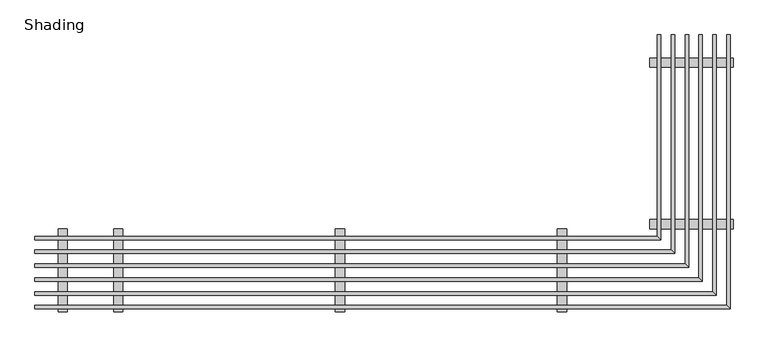
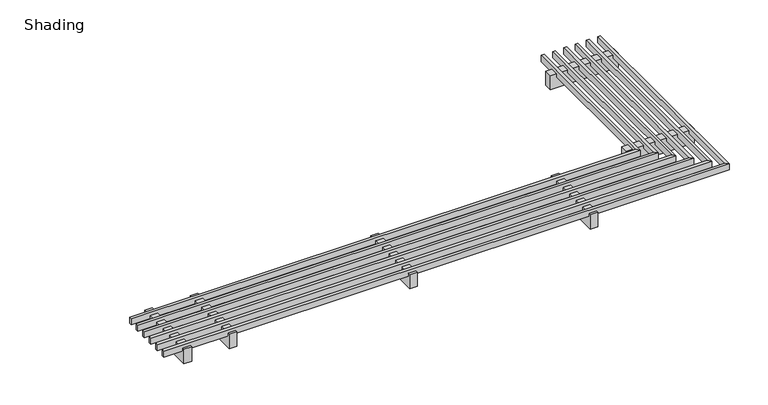
"""IFC4 building model written with IfcOpenShell, lengths in millimetres: railing geometry, Shading."""

from ifc_helpers import new_model, si_unit, frame, origin, place, context, project, spatial, polyline, outline, extrude, faceted_brep, source, transform, mapped, element, save


def shading_4c73cd6e(model_context):
    return source(origin(), model_context, "Body", "SolidModel", [
        faceted_brep([(-10644.3922358, -6454.4297826, 3702.05), (-10644.3922358, -6416.3297826, 3702.05), (-10644.3922358, -6416.3297826, 3613.15), (-10644.3922358, -6454.4297826, 3613.15), (-3005.3422358, -6454.4297826, 3613.15), (-3005.3422358, -6454.4297826, 3702.05), (-3043.4422358, -6416.3297826, 3613.15), (-3043.4422358, -6416.3297826, 3702.05), (-3005.3422358, -3438.1797826, 3702.05), (-3005.3422358, -3438.1797826, 3613.15), (-3043.4422358, -3438.1797826, 3613.15), (-3043.4422358, -3438.1797826, 3702.05)], [[[0, 1, 2, 3]], [[4, 5, 0, 3]], [[6, 4, 3, 2]], [[7, 6, 2, 1]], [[5, 7, 1, 0]], [[8, 9, 10, 11]], [[9, 8, 5, 4]], [[10, 9, 4, 6]], [[11, 10, 6, 7]], [[8, 11, 7, 5]]]),
        faceted_brep([(-10644.3922358, -6302.0297826, 3702.05), (-10644.3922358, -6263.9297826, 3702.05), (-10644.3922358, -6263.9297826, 3613.15), (-10644.3922358, -6302.0297826, 3613.15), (-3157.7422358, -6302.0297826, 3613.15), (-3157.7422358, -6302.0297826, 3702.05), (-3195.8422358, -6263.9297826, 3613.15), (-3195.8422358, -6263.9297826, 3702.05), (-3157.7422358, -3438.1797826, 3702.05), (-3157.7422358, -3438.1797826, 3613.15), (-3195.8422358, -3438.1797826, 3613.15), (-3195.8422358, -3438.1797826, 3702.05)], [[[0, 1, 2, 3]], [[4, 5, 0, 3]], [[6, 4, 3, 2]], [[7, 6, 2, 1]], [[5, 7, 1, 0]], [[8, 9, 10, 11]], [[9, 8, 5, 4]], [[10, 9, 4, 6]], [[11, 10, 6, 7]], [[8, 11, 7, 5]]]),
        faceted_brep([(-10644.3922358, -6149.6297826, 3702.05), (-10644.3922358, -6111.5297826, 3702.05), (-10644.3922358, -6111.5297826, 3613.15), (-10644.3922358, -6149.6297826, 3613.15), (-3310.1422358, -6149.6297826, 3613.15), (-3310.1422358, -6149.6297826, 3702.05), (-3348.2422358, -6111.5297826, 3613.15), (-3348.2422358, -6111.5297826, 3702.05), (-3310.1422358, -3438.1797826, 3702.05), (-3310.1422358, -3438.1797826, 3613.15), (-3348.2422358, -3438.1797826, 3613.15), (-3348.2422358, -3438.1797826, 3702.05)], [[[0, 1, 2, 3]], [[4, 5, 0, 3]], [[6, 4, 3, 2]], [[7, 6, 2, 1]], [[5, 7, 1, 0]], [[8, 9, 10, 11]], [[9, 8, 5, 4]], [[10, 9, 4, 6]], [[11, 10, 6, 7]], [[8, 11, 7, 5]]]),
        faceted_brep([(-10644.3922358, -5997.2297826, 3702.05), (-10644.3922358, -5959.1297826, 3702.05), (-10644.3922358, -5959.1297826, 3613.15), (-10644.3922358, -5997.2297826, 3613.15), (-3462.5422358, -5997.2297826, 3613.15), (-3462.5422358, -5997.2297826, 3702.05), (-3500.6422358, -5959.1297826, 3613.15), (-3500.6422358, -5959.1297826, 3702.05), (-3462.5422358, -3438.1797826, 3702.05), (-3462.5422358, -3438.1797826, 3613.15), (-3500.6422358, -3438.1797826, 3613.15), (-3500.6422358, -3438.1797826, 3702.05)], [[[0, 1, 2, 3]], [[4, 5, 0, 3]], [[6, 4, 3, 2]], [[7, 6, 2, 1]], [[5, 7, 1, 0]], [[8, 9, 10, 11]], [[9, 8, 5, 4]], [[10, 9, 4, 6]], [[11, 10, 6, 7]], [[8, 11, 7, 5]]]),
        faceted_brep([(-10644.3922358, -5844.8297826, 3702.05), (-10644.3922358, -5806.7297826, 3702.05), (-10644.3922358, -5806.7297826, 3613.15), (-10644.3922358, -5844.8297826, 3613.15), (-3614.9422358, -5844.8297826, 3613.15), (-3614.9422358, -5844.8297826, 3702.05), (-3653.0422358, -5806.7297826, 3613.15), (-3653.0422358, -5806.7297826, 3702.05), (-3614.9422358, -3438.1797826, 3702.05), (-3614.9422358, -3438.1797826, 3613.15), (-3653.0422358, -3438.1797826, 3613.15), (-3653.0422358, -3438.1797826, 3702.05)], [[[0, 1, 2, 3]], [[4, 5, 0, 3]], [[6, 4, 3, 2]], [[7, 6, 2, 1]], [[5, 7, 1, 0]], [[8, 9, 10, 11]], [[9, 8, 5, 4]], [[10, 9, 4, 6]], [[11, 10, 6, 7]], [[8, 11, 7, 5]]]),
        faceted_brep([(-10644.3922358, -5692.4297826, 3702.05), (-10644.3922358, -5654.3297826, 3702.05), (-10644.3922358, -5654.3297826, 3613.15), (-10644.3922358, -5692.4297826, 3613.15), (-3767.3422358, -5692.4297826, 3613.15), (-3767.3422358, -5692.4297826, 3702.05), (-3805.4422358, -5654.3297826, 3613.15), (-3805.4422358, -5654.3297826, 3702.05), (-3767.3422358, -3438.1797826, 3702.05), (-3767.3422358, -3438.1797826, 3613.15), (-3805.4422358, -3438.1797826, 3613.15), (-3805.4422358, -3438.1797826, 3702.05)], [[[0, 1, 2, 3]], [[4, 5, 0, 3]], [[6, 4, 3, 2]], [[7, 6, 2, 1]], [[5, 7, 1, 0]], [[8, 9, 10, 11]], [[9, 8, 5, 4]], [[10, 9, 4, 6]], [[11, 10, 6, 7]], [[8, 11, 7, 5]]]),
        extrude(outline(polyline([(-9679.1922358, -6486.1797826), (-9780.7922358, -6486.1797826), (-9780.7922358, -5571.7797826), (-9679.1922358, -5571.7797826), (-9679.1922358, -6486.1797826)])), frame((0.0, 0.0, 3454.4), z_axis=(0.0, 0.0, 1.0), x_axis=(1.0, 0.0, 0.0)), (0.0, 0.0, 1.0), 203.2),
        extrude(outline(polyline([(-7240.7922358, -6486.1797826), (-7342.3922358, -6486.1797826), (-7342.3922358, -5571.7797826), (-7240.7922358, -5571.7797826), (-7240.7922358, -6486.1797826)])), frame((0.0, 0.0, 3454.4), z_axis=(0.0, 0.0, 1.0), x_axis=(1.0, 0.0, 0.0)), (0.0, 0.0, 1.0), 203.2),
        extrude(outline(polyline([(-4802.3922358, -6486.1797826), (-4903.9922358, -6486.1797826), (-4903.9922358, -5571.7797826), (-4802.3922358, -5571.7797826), (-4802.3922358, -6486.1797826)])), frame((0.0, 0.0, 3454.4), z_axis=(0.0, 0.0, 1.0), x_axis=(1.0, 0.0, 0.0)), (0.0, 0.0, 1.0), 203.2),
        extrude(outline(polyline([(-2973.5922358, -5470.1797826), (-2973.5922358, -5571.7797826), (-3887.9922358, -5571.7797826), (-3887.9922358, -5470.1797826), (-2973.5922358, -5470.1797826)])), frame((0.0, 0.0, 3454.4), z_axis=(0.0, 0.0, 1.0), x_axis=(1.0, 0.0, 0.0)), (0.0, 0.0, 1.0), 203.2),
        extrude(outline(polyline([(-10288.7922358, -6486.1797826), (-10390.3922358, -6486.1797826), (-10390.3922358, -5571.7797826), (-10288.7922358, -5571.7797826), (-10288.7922358, -6486.1797826)])), frame((0.0, 0.0, 3454.4), z_axis=(0.0, 0.0, 1.0), x_axis=(1.0, 0.0, 0.0)), (0.0, 0.0, 1.0), 203.2),
        extrude(outline(polyline([(-2973.5922358, -3692.1797826), (-2973.5922358, -3793.7797826), (-3887.9922358, -3793.7797826), (-3887.9922358, -3692.1797826), (-2973.5922358, -3692.1797826)])), frame((0.0, 0.0, 3454.4), z_axis=(0.0, 0.0, 1.0), x_axis=(1.0, 0.0, 0.0)), (0.0, 0.0, 1.0), 203.2),
    ])


if __name__ == "__main__":
    model = new_model("IFC4")
    model_context = context("Model", 3, world=origin())
    ifc_project = project(units=[si_unit("LENGTHUNIT", "METRE", prefix="MILLI")], contexts=[model_context])
    site = spatial("IfcSite", under=ifc_project)
    building = spatial("IfcBuilding", under=site)
    placement = place(None, origin())
    shading_shape = shading_4c73cd6e(model_context)
    element("IfcRailing", 1, ObjectType="Shading", at=placement, inside=building, context=model_context, shape_type="MappedRepresentation", body=[
        mapped(shading_shape, transform((0.0, 0.0, 0.0), x_axis=(1.0, 0.0, 0.0), y_axis=(0.0, 1.0, 0.0), z_axis=(0.0, 0.0, 1.0))),
    ])
    save(model, "model.ifc")

# Revit data of these elements
# Element 1 (IfcRailing, "Shading")
#   Materials on its faces: "Wood - Teak"
# Materials
#   "Wood - Teak": class "Wood", colour RGB 169 114 85, transparency 0, Cost = 0
